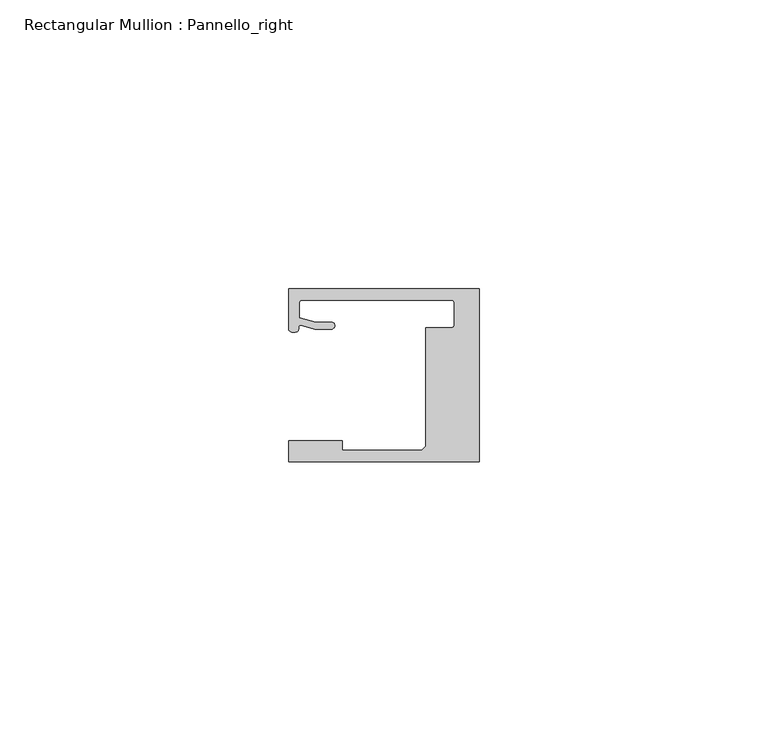
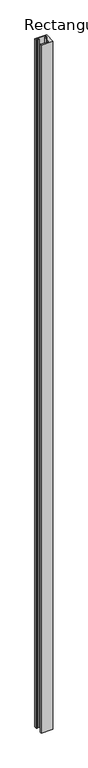
"""IFC4 building model written with IfcOpenShell, lengths in millimetres: member geometry, Rectangular Mullion : Pannello_right."""

import ifcopenshell
import ifcopenshell.guid

model = None  # the IFC model being written
_history = None  # IfcOwnerHistory: only IFC2X3 demands one
_inside = {}  # id of a spatial element -> (the spatial element, [elements in it])
_under = {}  # id of a project, library or spatial element -> (it, [spatial elements below it])
_declared = {}  # id of a project -> (the project, [libraries it declares])
_typed = {}  # id of a type object -> (the type object, [elements of that type])
_made_of = {}  # id of a material, layer set ... -> (it, [elements and type objects made of it])


def new_model(schema):
    """Start an empty IFC model of exactly this schema.

    Asked for "IFC4X3", IfcOpenShell would pick the latest addendum, in which some entities
    have other attributes; the version numbers below select the first issue.
    IFC2X3 requires an IfcOwnerHistory on every rooted entity: one is made here for all.
    """
    global model, _history
    if schema == "IFC4X3":
        model = ifcopenshell.file(schema_version=(4, 3, 0, 0))
    else:
        model = ifcopenshell.file(schema=schema)
    _inside.clear()
    _under.clear()
    _declared.clear()
    _typed.clear()
    _made_of.clear()
    _history = None
    if model.schema == "IFC2X3":
        org = make("IfcOrganization", Name="unknown")
        user = make(
            "IfcPersonAndOrganization",
            ThePerson=make("IfcPerson", FamilyName="unknown"),
            TheOrganization=org,
        )
        app = make(
            "IfcApplication",
            ApplicationDeveloper=org,
            Version="unknown",
            ApplicationFullName="unknown",
            ApplicationIdentifier="unknown",
        )
        _history = make(
            "IfcOwnerHistory",
            OwningUser=user,
            OwningApplication=app,
            ChangeAction="ADDED",
            CreationDate=0,
        )
    return model


def make(cls, **values):
    """One entity of the class cls with the attributes given. An attribute that is None is left unset."""
    return model.create_entity(
        cls, **{name: value for name, value in values.items() if value is not None}
    )


def rooted(cls, **values):
    """An entity with a GlobalId (a new one), such as an element, a storey or a relation."""
    return make(cls, GlobalId=ifcopenshell.guid.new(), OwnerHistory=_history, **values)


def si_unit(unit_type, name, prefix=None):
    """IfcSIUnit, for example si_unit("LENGTHUNIT", "METRE", prefix="MILLI")."""
    return make("IfcSIUnit", UnitType=unit_type, Prefix=prefix, Name=name)


def assignment(units):
    """IfcUnitAssignment: the units of a project."""
    return None if units is None else make("IfcUnitAssignment", Units=units)


def point(xyz):
    """IfcCartesianPoint."""
    return None if xyz is None else make("IfcCartesianPoint", Coordinates=xyz)


def direction(xyz):
    """IfcDirection."""
    return None if xyz is None else make("IfcDirection", DirectionRatios=xyz)


def frame(location, z_axis=None, x_axis=None):
    """IfcAxis2Placement3D, a coordinate frame: its origin and axes. An axis left out is left unset."""
    return make(
        "IfcAxis2Placement3D",
        Location=point(location),
        Axis=direction(z_axis),
        RefDirection=direction(x_axis),
    )


def origin():
    """The frame at (0, 0, 0) with its axes left unset."""
    return frame((0.0, 0.0, 0.0))


def place(relative_to, where):
    """IfcLocalPlacement: puts the frame where relative to a parent placement (None: the world)."""
    return make(
        "IfcLocalPlacement", PlacementRelTo=relative_to, RelativePlacement=where
    )


def context(
    kind, dimensions, precision=None, world=None, true_north=None, identifier=None
):
    """IfcGeometricRepresentationContext, for example the 3D "Model" context."""
    return make(
        "IfcGeometricRepresentationContext",
        ContextIdentifier=identifier,
        ContextType=kind,
        CoordinateSpaceDimension=dimensions,
        Precision=precision,
        WorldCoordinateSystem=world,
        TrueNorth=true_north,
    )


def project(units=None, contexts=None):
    """IfcProject with its units and contexts."""
    return rooted(
        "IfcProject",
        Name="project",
        RepresentationContexts=contexts,
        UnitsInContext=assignment(units),
    )


def spatial(cls, under=None, at=None, **own):
    """A site, building, storey or space (cls), placed at a placement, below another one or the project."""
    s = rooted(cls, ObjectPlacement=at, **own)
    if under is not None:
        _under.setdefault(under.id(), (under, []))[1].append(s)
    return s


def polyline(points):
    """IfcPolyline through the points."""
    return make("IfcPolyline", Points=[point(p) for p in points])


def circle_curve(where, radius):
    """IfcCircle in the frame where."""
    return make("IfcCircle", Position=where, Radius=radius)


def shape(context_of_items, identifier, shape_type, items):
    """IfcShapeRepresentation: the items that make up one representation, for example the "Body"."""
    return make(
        "IfcShapeRepresentation",
        ContextOfItems=context_of_items,
        RepresentationIdentifier=identifier,
        RepresentationType=shape_type,
        Items=items,
    )


def source(mapping_origin, context_of_items, identifier, shape_type, items):
    """IfcRepresentationMap: a shape defined once, which mapped items show again and again."""
    return make(
        "IfcRepresentationMap",
        MappingOrigin=mapping_origin,
        MappedRepresentation=shape(context_of_items, identifier, shape_type, items),
    )


def transform(
    local_origin,
    x_axis=None,
    y_axis=None,
    z_axis=None,
    scale=None,
    scale2=None,
    scale3=None,
    uniform=True,
):
    """IfcCartesianTransformationOperator3D, or its non-uniform kind. x_axis, y_axis, z_axis: its Axis1, 2, 3."""
    if uniform:
        return make(
            "IfcCartesianTransformationOperator3D",
            Axis1=direction(x_axis),
            Axis2=direction(y_axis),
            LocalOrigin=point(local_origin),
            Scale=scale,
            Axis3=direction(z_axis),
        )
    return make(
        "IfcCartesianTransformationOperator3DnonUniform",
        Axis1=direction(x_axis),
        Axis2=direction(y_axis),
        LocalOrigin=point(local_origin),
        Scale=scale,
        Axis3=direction(z_axis),
        Scale2=scale2,
        Scale3=scale3,
    )


def mapped(mapping_source, mapping_target):
    """IfcMappedItem: shows the shape of a source again, moved by a transform."""
    return make(
        "IfcMappedItem", MappingSource=mapping_source, MappingTarget=mapping_target
    )


def made_of(thing, what):
    """Note that an element or type object is made of a material, layer set ...; save() writes the relation."""
    if what is not None:
        _made_of.setdefault(what.id(), (what, []))[1].append(thing)
    return thing


def element(
    cls,
    number,
    at=None,
    inside=None,
    cuts=None,
    type_object=None,
    material=None,
    context=None,
    identifier="Body",
    shape_type=None,
    held_by="IfcProductDefinitionShape",
    body=None,
    shapes=None,
    **own,
):
    """One element of the class cls, such as IfcWall. Its Tag is "e" and its number.

    at: its placement. inside: the storey or other place that contains it. cuts: it is an
    opening in that element (IfcRelVoidsElement). A single representation is given by context,
    identifier, shape_type and body (its items); several are given by shapes. held_by: the class
    of the entity that holds the representations. save() writes the other relations.
    """
    e = rooted(cls, Tag="e%d" % number, ObjectPlacement=at, **own)
    if body is not None:
        shapes = [shape(context, identifier, shape_type, body)]
    if shapes is not None:
        e.Representation = make(held_by, Representations=shapes)
    if inside is not None:
        _inside.setdefault(inside.id(), (inside, []))[1].append(e)
    if cuts is not None:
        rooted(
            "IfcRelVoidsElement", RelatingBuildingElement=cuts, RelatedOpeningElement=e
        )
    if type_object is not None:
        _typed.setdefault(type_object.id(), (type_object, []))[1].append(e)
    return made_of(e, material)


def aggregate(whole, parts):
    """IfcRelAggregates: a whole, such as a stair, and the parts it consists of."""
    return rooted("IfcRelAggregates", RelatingObject=whole, RelatedObjects=parts)


def save(model, path):
    """Write the relations noted so far, then the file.

    IfcRelAggregates (storeys below a building ...), IfcRelContainedInSpatialStructure (elements
    in a storey), IfcRelDefinesByType, IfcRelAssociatesMaterial and IfcRelDeclares: one each for
    every whole, place, type object, material and project.
    """
    for whole, parts in _under.values():
        aggregate(whole, parts)
    for where, things in _inside.values():
        rooted(
            "IfcRelContainedInSpatialStructure",
            RelatedElements=things,
            RelatingStructure=where,
        )
    for kind, things in _typed.values():
        rooted("IfcRelDefinesByType", RelatedObjects=things, RelatingType=kind)
    for what, things in _made_of.values():
        rooted("IfcRelAssociatesMaterial", RelatedObjects=things, RelatingMaterial=what)
    for by, libraries in _declared.values():
        rooted("IfcRelDeclares", RelatingContext=by, RelatedDefinitions=libraries)
    model.write(path)


def plane_surface(at):
    """IfcPlane: the flat surface through the origin of the frame at, square to its z axis."""
    return make("IfcPlane", Position=at)


def cylinder_surface(at, radius):
    """IfcCylindricalSurface: all points at the distance radius from the z axis of the frame at."""
    return make("IfcCylindricalSurface", Position=at, Radius=radius)


def revolved_surface(curve, axis_point, axis_direction):
    """IfcSurfaceOfRevolution: the curve turned about the line through axis_point along axis_direction."""
    return make(
        "IfcSurfaceOfRevolution",
        SweptCurve=make("IfcArbitraryOpenProfileDef", ProfileType="CURVE", Curve=curve),
        AxisPosition=make("IfcAxis1Placement", Location=point(axis_point), Axis=direction(axis_direction)),
    )


def extruded_surface(curve, direction_of_extrusion, depth):
    """IfcSurfaceOfLinearExtrusion: the curve pushed along a direction by depth."""
    return make(
        "IfcSurfaceOfLinearExtrusion",
        SweptCurve=make("IfcArbitraryOpenProfileDef", ProfileType="CURVE", Curve=curve),
        ExtrudedDirection=direction(direction_of_extrusion),
        Depth=depth,
    )


def spline_curve(degree, points, multiplicities, knots, weights=None):
    """IfcBSplineCurveWithKnots; with weights, IfcRationalBSplineCurveWithKnots."""
    own = dict(
        Degree=degree,
        ControlPointsList=[point(p) for p in points],
        CurveForm="UNSPECIFIED",
        ClosedCurve=False,
        SelfIntersect=False,
        KnotMultiplicities=multiplicities,
        Knots=knots,
        KnotSpec="UNSPECIFIED",
    )
    if weights is None:
        return make("IfcBSplineCurveWithKnots", **own)
    return make("IfcRationalBSplineCurveWithKnots", WeightsData=weights, **own)


def advanced_brep(points, edges, surfaces, faces):
    """IfcAdvancedBrep: a solid bounded by faces that lie on surfaces and meet in shared edges.

    An edge is (start, end): straight between two places in points (the first is 0);
    or (start, end, curve); or (start, end, curve, False) where it runs against its curve.
    A face is (place in surfaces, loops), or (place, loops, False) where it looks against
    its surface's normal. A loop lists edges by number (the first is 1), with a minus sign
    where the edge is run from its end to its start. The first loop is the outer one.
    """
    corners = [point(p) for p in points]
    vertices = [make("IfcVertexPoint", VertexGeometry=c) for c in corners]
    made = []
    for start, end, *more in edges:
        made.append(
            make(
                "IfcEdgeCurve",
                EdgeStart=vertices[start],
                EdgeEnd=vertices[end],
                EdgeGeometry=more[0] if more else make("IfcPolyline", Points=[corners[start], corners[end]]),
                SameSense=more[1] if len(more) > 1 else True,
            )
        )
    hull = []
    for where, loops, *sense in faces:
        bounds = []
        for j, loop in enumerate(loops):
            ring = [make("IfcOrientedEdge", EdgeElement=made[abs(k) - 1], Orientation=k > 0) for k in loop]
            bounds.append(
                make(
                    "IfcFaceOuterBound" if j == 0 else "IfcFaceBound",
                    Bound=make("IfcEdgeLoop", EdgeList=ring),
                    Orientation=True,
                )
            )
        hull.append(make("IfcAdvancedFace", Bounds=bounds, FaceSurface=surfaces[where], SameSense=sense[0] if sense else True))
    return make("IfcAdvancedBrep", Outer=make("IfcClosedShell", CfsFaces=hull))


def rectangular_mullion_pannello_right_f5c28175(model_context):
    return source(origin(), model_context, "Body", "AdvancedBrep", [
        advanced_brep(
        [(-33.0, -15.0, 0.0), (0.0, -15.0, 0.0), (0.0, 15.0, 0.0), (-33.0000135, 15.0, 0.0), (-33.0000135, 8.0000472, 0.0), (-30.9223017, 8.6490241, 0.0), (-28.4999305, 7.9999523, 0.0), (-25.59998, 7.9999523, 0.0), (-25.59998, 9.1999523, 0.0), (-28.3419477, 9.1999523, 0.0), (-31.19998, 9.9657591, 0.0), (-31.19998, 12.50001, 0.0), (-30.69998, 13.00001, 0.0), (-4.7999726, 13.00001, 0.0), (-4.2999726, 12.50001, 0.0), (-4.2999726, 8.7500595, 0.0), (-4.7999726, 8.2500595, 0.0), (-9.2999726, 8.2500595, 0.0), (-9.2999726, -12.2999849, 0.0), (-10.0000103, -13.0000004, 0.0), (-23.700041, -13.0000004, 0.0), (-23.700041, -11.3000004, 0.0), (-33.0, -11.3000004, 0.0), (-33.0, -15.0, -2026.9999865), (-33.0, -11.3000004, -2026.9999865), (-23.700041, -11.3000004, -2026.9999865), (-23.700041, -13.0000004, -2026.9999865), (-10.0000103, -13.0000004, -2026.9999865), (-9.2999726, -12.2999849, -2026.9999865), (-9.2999726, 8.2500595, -2026.9999865), (-4.7999726, 8.2500595, -2026.9999865), (-4.2999726, 8.7500595, -2026.9999865), (-4.2999726, 12.50001, -2026.9999865), (-4.7999726, 13.00001, -2026.9999865), (-30.69998, 13.00001, -2026.9999865), (-31.19998, 12.50001, -2026.9999865), (-31.19998, 9.9657591, -2026.9999865), (-28.3419477, 9.1999523, -2026.9999865), (-25.59998, 9.1999523, -2026.9999865), (-25.59998, 7.9999523, -2026.9999865), (-28.4999305, 7.9999523, -2026.9999865), (-30.9223017, 8.6490241, -2026.9999865), (-33.0000135, 8.0000472, -2026.9999865), (-33.0000135, 15.0, -2026.9999865), (0.0, 15.0, -2026.9999865), (0.0, -15.0, -2026.9999865)],
        [
            (0, 1),
            (1, 2),
            (2, 3),
            (3, 4),
            (4, 5, spline_curve(3, [(-33.0000135, 8.0000472, 0.0), (-33.0000135, 7.457047519, 0.0), (-32.262327879, 7.456527435, 0.0), (-31.357433266, 7.563996614, 0.0), (-31.305645054, 7.690065204, 0.0), (-31.298563602, 8.366228555, 0.0), (-31.312054066, 8.717747958, 0.0), (-30.9223017, 8.6490241, 0.0)], [4, 2, 2, 4], [0.0, 0.0027053965905959043, 0.0058611956533709, 0.007702013405570312])),
            (5, 6),
            (6, 7),
            (7, 8, circle_curve(frame((-25.59998, 8.5999523, 0.0), z_axis=(0.0, 0.0, 1.0), x_axis=(0.0, 1.0, 0.0)), 0.6)),
            (8, 9),
            (9, 10),
            (10, 11),
            (11, 12, circle_curve(frame((-30.69998, 12.50001, 0.0), z_axis=(0.0, 0.0, -1.0), x_axis=(0.0, 1.0, 0.0)), 0.5)),
            (12, 13),
            (13, 14, circle_curve(frame((-4.7999726, 12.50001, 0.0), z_axis=(0.0, 0.0, -1.0), x_axis=(1.0, 0.0, 0.0)), 0.5)),
            (14, 15),
            (15, 16, circle_curve(frame((-4.7999726, 8.7500595, 0.0), z_axis=(0.0, 0.0, -1.0), x_axis=(0.0, -1.0, 0.0)), 0.5)),
            (16, 17),
            (17, 18),
            (18, 19),
            (19, 20),
            (20, 21),
            (21, 22),
            (22, 0),
            (23, 24),
            (24, 25),
            (25, 26),
            (26, 27),
            (27, 28),
            (28, 29),
            (29, 30),
            (30, 31, circle_curve(frame((-4.7999726, 8.7500595, -2026.9999865), z_axis=(0.0, 0.0, 1.0), x_axis=(0.0, -1.0, 0.0)), 0.5)),
            (31, 32),
            (32, 33, circle_curve(frame((-4.7999726, 12.50001, -2026.9999865), z_axis=(0.0, 0.0, 1.0), x_axis=(1.0, 0.0, 0.0)), 0.5)),
            (33, 34),
            (34, 35, circle_curve(frame((-30.69998, 12.50001, -2026.9999865), z_axis=(0.0, 0.0, 1.0), x_axis=(0.0, 1.0, 0.0)), 0.5)),
            (35, 36),
            (36, 37),
            (37, 38),
            (38, 39, circle_curve(frame((-25.59998, 8.5999523, -2026.9999865), z_axis=(0.0, 0.0, -1.0), x_axis=(0.0, 1.0, 0.0)), 0.6)),
            (39, 40),
            (40, 41),
            (41, 42, spline_curve(3, [(-30.9223017, 8.6490241, -2026.9999865), (-31.312054066, 8.717747958, -2026.9999865), (-31.298563602, 8.366228555, -2026.9999865), (-31.305645054, 7.690065204, -2026.9999865), (-31.357433266, 7.563996614, -2026.9999865), (-32.262327879, 7.456527435, -2026.9999865), (-33.0000135, 7.457047519, -2026.9999865), (-33.0000135, 8.0000472, -2026.9999865)], [4, 2, 2, 4], [0.0, 0.001840817752199412, 0.004996616814974408, 0.007702013405570312])),
            (42, 43),
            (43, 44),
            (44, 45),
            (45, 23),
            (0, 23),
            (45, 1),
            (44, 2),
            (43, 3),
            (42, 4),
            (41, 5),
            (40, 6),
            (39, 7),
            (38, 8),
            (37, 9),
            (36, 10),
            (35, 11),
            (34, 12),
            (33, 13),
            (32, 14),
            (31, 15),
            (30, 16),
            (29, 17),
            (28, 18),
            (27, 19),
            (26, 20),
            (25, 21),
            (24, 22),
        ],
        [
            plane_surface(frame((0.0, -36.2491502, 0.0), z_axis=(0.0, 0.0, 1.0), x_axis=(-1.0, 0.0, 0.0))),
            plane_surface(frame((0.0, -36.2491502, -2026.9999865), z_axis=(0.0, 0.0, -1.0), x_axis=(-1.0, 0.0, 0.0))),
            plane_surface(frame((-33.0, -15.0, 0.0), z_axis=(0.0, -1.0, 0.0), x_axis=(0.0, 0.0, -1.0))),
            plane_surface(frame((0.0, -15.0, 0.0), z_axis=(1.0, 0.0, 0.0), x_axis=(0.0, 0.0, -1.0))),
            plane_surface(frame((0.0, 15.0, 0.0), z_axis=(0.0, 1.0, 0.0), x_axis=(0.0, 0.0, -1.0))),
            plane_surface(frame((-33.0000135, 15.0, 0.0), z_axis=(-1.0, 0.0, 0.0), x_axis=(0.0, 0.0, -1.0))),
            extruded_surface(spline_curve(3, [(-33.0000135, 8.0000472, -2026.9999865), (-33.0000135, 7.457047519, -2026.9999865), (-32.262327879, 7.456527435, -2026.9999865), (-31.357433266, 7.563996614, -2026.9999865), (-31.305645054, 7.690065204, -2026.9999865), (-31.298563602, 8.366228555, -2026.9999865), (-31.312054066, 8.717747958, -2026.9999865), (-30.9223017, 8.6490241, -2026.9999865)], [4, 2, 2, 4], [0.0, 0.0027053965905959043, 0.0058611956533709, 0.007702013405570312]), (0.0, 0.0, 2026.9999865), 2026.9999865),
            plane_surface(frame((-30.9223017, 8.6490241, 0.0), z_axis=(-0.2588188320019168, -0.965925883389178, 0.0), x_axis=(0.0, 0.0, -1.0))),
            plane_surface(frame((-28.4999305, 7.9999523, 0.0), z_axis=(0.0, -1.0, 0.0), x_axis=(0.0, 0.0, -1.0))),
            cylinder_surface(frame((-25.59998, 8.5999523, 0.0), z_axis=(0.0, 0.0, 1.0), x_axis=(0.0, 1.0, 0.0)), 0.6),
            plane_surface(frame((-25.59998, 9.1999523, 0.0), z_axis=(0.0, 1.0, 0.0), x_axis=(0.0, 0.0, -1.0))),
            plane_surface(frame((-28.3419477, 9.1999523, 0.0), z_axis=(0.2588188320428738, 0.9659258833782035, 0.0), x_axis=(0.0, 0.0, -1.0))),
            plane_surface(frame((-31.19998, 9.9657591, 0.0), z_axis=(1.0, 0.0, 0.0), x_axis=(0.0, 0.0, -1.0))),
            revolved_surface(polyline([(-30.69998, 13.00001, -2026.9999865), (-30.69998, 13.00001, 0.0)]), (-30.69998, 12.50001, 0.0), (0.0, 0.0, -1.0)),
            plane_surface(frame((-30.69998, 13.00001, 0.0), z_axis=(0.0, -1.0, 0.0), x_axis=(0.0, 0.0, -1.0))),
            revolved_surface(polyline([(-4.2999726, 12.50001, -2026.9999865), (-4.2999726, 12.50001, 0.0)]), (-4.7999726, 12.50001, 0.0), (0.0, 0.0, -1.0)),
            plane_surface(frame((-4.2999726, 12.50001, 0.0), z_axis=(-1.0, 0.0, 0.0), x_axis=(0.0, 0.0, -1.0))),
            revolved_surface(polyline([(-4.7999726, 8.2500595, -2026.9999865), (-4.7999726, 8.2500595, 0.0)]), (-4.7999726, 8.7500595, 0.0), (0.0, 0.0, -1.0)),
            plane_surface(frame((-4.7999726, 8.2500595, 0.0), z_axis=(0.0, 1.0, 0.0), x_axis=(0.0, 0.0, -1.0))),
            plane_surface(frame((-9.2999726, 8.2500595, 0.0), z_axis=(-1.0, 0.0, 0.0), x_axis=(0.0, 0.0, -1.0))),
            plane_surface(frame((-9.2999726, -12.2999849, 0.0), z_axis=(-0.7070955486278075, 0.7071180135668587, 0.0), x_axis=(0.0, 0.0, -1.0))),
            plane_surface(frame((-10.0000103, -13.0000004, 0.0), z_axis=(0.0, 1.0, 0.0), x_axis=(0.0, 0.0, -1.0))),
            plane_surface(frame((-23.700041, -13.0000004, 0.0), z_axis=(1.0, 0.0, 0.0), x_axis=(0.0, 0.0, -1.0))),
            plane_surface(frame((-23.700041, -11.3000004, 0.0), z_axis=(0.0, 1.0, 0.0), x_axis=(0.0, 0.0, -1.0))),
            plane_surface(frame((-33.0, -11.3000004, 0.0), z_axis=(-1.0, 0.0, 0.0), x_axis=(0.0, 0.0, -1.0))),
        ],
        [
            (0, [[1, 2, 3, 4, 5, 6, 7, 8, 9, 10, 11, 12, 13, 14, 15, 16, 17, 18, 19, 20, 21, 22, 23]]),
            (1, [[24, 25, 26, 27, 28, 29, 30, 31, 32, 33, 34, 35, 36, 37, 38, 39, 40, 41, 42, 43, 44, 45, 46]]),
            (2, [[-1, 47, -46, 48]]),
            (3, [[-2, -48, -45, 49]]),
            (4, [[-3, -49, -44, 50]]),
            (5, [[-4, -50, -43, 51]]),
            (6, [[-5, -51, -42, 52]]),
            (7, [[-6, -52, -41, 53]]),
            (8, [[-7, -53, -40, 54]]),
            (9, [[-8, -54, -39, 55]]),
            (10, [[-9, -55, -38, 56]]),
            (11, [[-10, -56, -37, 57]]),
            (12, [[-11, -57, -36, 58]]),
            (13, [[-12, -58, -35, 59]]),
            (14, [[-13, -59, -34, 60]]),
            (15, [[-14, -60, -33, 61]]),
            (16, [[-15, -61, -32, 62]]),
            (17, [[-16, -62, -31, 63]]),
            (18, [[-17, -63, -30, 64]]),
            (19, [[-18, -64, -29, 65]]),
            (20, [[-19, -65, -28, 66]]),
            (21, [[-20, -66, -27, 67]]),
            (22, [[-21, -67, -26, 68]]),
            (23, [[-22, -68, -25, 69]]),
            (24, [[-23, -69, -24, -47]]),
        ],
    ),
    ])


if __name__ == "__main__":
    model = new_model("IFC4")
    model_context = context("Model", 3, world=origin())
    ifc_project = project(units=[si_unit("LENGTHUNIT", "METRE", prefix="MILLI")], contexts=[model_context])
    site = spatial("IfcSite", under=ifc_project)
    building = spatial("IfcBuilding", under=site)
    placement = place(None, origin())
    rectangular_mullion_pannello_right_shape = rectangular_mullion_pannello_right_f5c28175(model_context)
    element("IfcMember", 1, ObjectType="Rectangular Mullion : Pannello_right", at=placement, inside=building, context=model_context, shape_type="MappedRepresentation", body=[
        mapped(rectangular_mullion_pannello_right_shape, transform((0.0, 0.0, 0.0), x_axis=(1.0, 0.0, 0.0), y_axis=(0.0, 1.0, 0.0), z_axis=(0.0, 0.0, 1.0))),
    ])
    save(model, "model.ifc")

# Revit data of these elements
# Type "Rectangular Mullion : Pannello_right"
#   built-in parameter 1007322 = 0.0984252 (stored number, unit not read)
#   built-in parameter 1007321 = 0.0305117 (stored number, unit not read)
#   built-in parameter 1007320 = 0 (stored number, unit not read)
